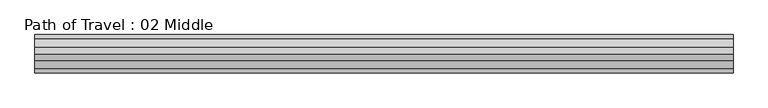
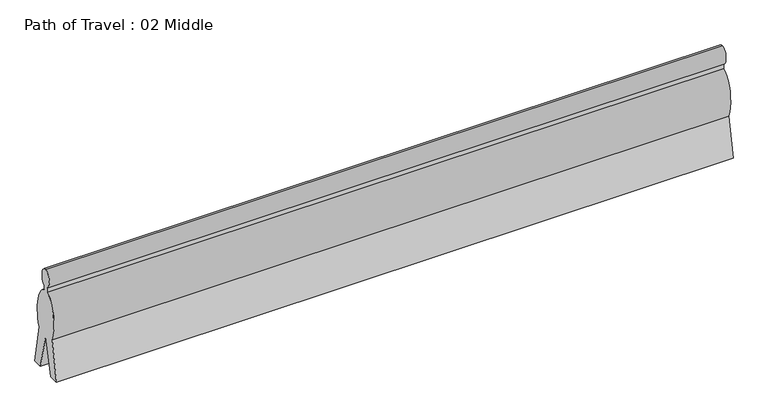
"""IFC4 building model written with IfcOpenShell, lengths in millimetres: proxy geometry, Path of Travel : 02 Middle."""

from ifc_helpers import new_model, si_unit, point, frame, origin, place, context, project, spatial, ellipse_curve, trimmed, source, transform, mapped, element, save
from ifc_brep_helpers import plane_surface, extruded_surface, advanced_brep


def path_of_travel_02_middle_3282dce8(model_context):
    return source(origin(), model_context, "Body", "AdvancedBrep", [
        advanced_brep(
        [(227.5554837, 0.0, 1727.2), (227.5554837, 42.9018657, 1436.6534209), (227.5554837, 42.9018657, 1363.4763406), (227.5554837, 184.1186263, 643.4144547), (227.5554837, 297.5699544, 0.0), (227.5554837, 145.6574193, 0.0), (227.5554837, 0.0, 584.2), (227.5554837, -145.6574193, 0.0), (227.5554837, -297.5699544, 0.0), (227.5554837, -184.1186263, 643.4144547), (227.5554837, -42.9018657, 1363.4763406), (227.5554837, -42.9018657, 1436.6534209), (11047.9554837, 0.0, 1727.2), (11047.9554837, -42.9018657, 1436.6534209), (11047.9554837, -42.9018657, 1363.4763406), (11047.9554837, -184.1186263, 643.4144547), (11047.9554837, -297.5699544, 0.0), (11047.9554837, -145.6574193, 0.0), (11047.9554837, 0.0, 584.2), (11047.9554837, 145.6574193, 0.0), (11047.9554837, 297.5699544, 0.0), (11047.9554837, 184.1186263, 643.4144547), (11047.9554837, 42.9018657, 1363.4763406), (11047.9554837, 42.9018657, 1436.6534209)],
        [
            (0, 1, ellipse_curve(frame((227.5554837, 0.0, 1574.8), z_axis=(-1.0, 0.0, 0.0), x_axis=(0.0, 0.0, 1.0)), 152.4, 101.6)),
            (1, 2),
            (2, 3, ellipse_curve(frame((227.5554837, 0.0, 914.4), z_axis=(-1.0, 0.0, 0.0), x_axis=(0.0, 0.0, -1.0)), 457.2, 228.6)),
            (3, 4),
            (4, 5),
            (5, 6),
            (6, 7),
            (7, 8),
            (8, 9),
            (9, 10, ellipse_curve(frame((227.5554837, 0.0, 914.4), z_axis=(-1.0, 0.0, 0.0), x_axis=(0.0, 0.0, -1.0)), 457.2, 228.6)),
            (10, 11),
            (11, 0, ellipse_curve(frame((227.5554837, 0.0, 1574.8), z_axis=(-1.0, 0.0, 0.0), x_axis=(0.0, 0.0, 1.0)), 152.4, 101.6)),
            (12, 13, ellipse_curve(frame((11047.9554837, 0.0, 1574.8), z_axis=(1.0, 0.0, 0.0), x_axis=(0.0, 0.0, 1.0)), 152.4, 101.6)),
            (13, 14),
            (14, 15, ellipse_curve(frame((11047.9554837, 0.0, 914.4), z_axis=(1.0, 0.0, 0.0), x_axis=(0.0, 0.0, -1.0)), 457.2, 228.6)),
            (15, 16),
            (16, 17),
            (17, 18),
            (18, 19),
            (19, 20),
            (20, 21),
            (21, 22, ellipse_curve(frame((11047.9554837, 0.0, 914.4), z_axis=(1.0, 0.0, 0.0), x_axis=(0.0, 0.0, -1.0)), 457.2, 228.6)),
            (22, 23),
            (23, 12, ellipse_curve(frame((11047.9554837, 0.0, 1574.8), z_axis=(1.0, 0.0, 0.0), x_axis=(0.0, 0.0, 1.0)), 152.4, 101.6)),
            (0, 12),
            (23, 1),
            (22, 2),
            (21, 3),
            (20, 4),
            (19, 5),
            (18, 6),
            (17, 7),
            (16, 8),
            (15, 9),
            (14, 10),
            (13, 11),
        ],
        [
            plane_surface(frame((227.5554837, 0.0, 0.0), z_axis=(-1.0, 0.0, 0.0), x_axis=(0.0, 0.0, 1.0))),
            plane_surface(frame((11047.9554837, 0.0, 0.0), z_axis=(1.0, 0.0, 0.0), x_axis=(0.0, 0.0, 1.0))),
            extruded_surface(trimmed(ellipse_curve(frame((11047.9554837, 0.0, 1574.8), z_axis=(-1.0, 0.0, 0.0), x_axis=(0.0, 0.0, 1.0)), 152.4, 101.6), [point((11047.9554837, 0.0, 1727.2))], [point((11047.9554837, 42.9018657, 1436.6534209))], True, "CARTESIAN"), (-10820.4, 0.0, 0.0), 10820.4),
            plane_surface(frame((227.5554837, 42.9018657, 1436.6534209), z_axis=(0.0, 1.0, 0.0), x_axis=(1.0, 0.0, 0.0))),
            extruded_surface(trimmed(ellipse_curve(frame((11047.9554837, 0.0, 914.4), z_axis=(-1.0, 0.0, 0.0), x_axis=(0.0, 0.0, -1.0)), 457.2, 228.6), [point((11047.9554837, 42.9018657, 1363.4763406))], [point((11047.9554837, 184.1186263, 643.4144547))], True, "CARTESIAN"), (-10820.4, 0.0, 0.0), 10820.4),
            plane_surface(frame((227.5554837, 184.1186263, 643.4144547), z_axis=(0.0, 0.9848077530122078, 0.17364817766693205), x_axis=(1.0, 0.0, 0.0))),
            plane_surface(frame((227.5554837, 297.5699544, 0.0), z_axis=(0.0, 0.0, -1.0), x_axis=(1.0, 0.0, 0.0))),
            plane_surface(frame((227.5554837, 145.6574193, 0.0), z_axis=(0.0, -0.9702957262760199, -0.2419218955995739), x_axis=(1.0, 0.0, 0.0))),
            plane_surface(frame((227.5554837, 0.0, 584.2), z_axis=(0.0, 0.9702957262759961, -0.24192189559966923), x_axis=(1.0, 0.0, 0.0))),
            plane_surface(frame((227.5554837, -145.6574193, 0.0), z_axis=(0.0, 0.0, -1.0), x_axis=(1.0, 0.0, 0.0))),
            plane_surface(frame((227.5554837, -297.5699544, 0.0), z_axis=(0.0, -0.984807753012208, 0.17364817766693066), x_axis=(1.0, 0.0, 0.0))),
            extruded_surface(trimmed(ellipse_curve(frame((11047.9554837, 0.0, 914.4), z_axis=(-1.0, 0.0, 0.0), x_axis=(0.0, 0.0, -1.0)), 457.2, 228.6), [point((11047.9554837, -184.1186263, 643.4144547))], [point((11047.9554837, -42.9018657, 1363.4763406))], True, "CARTESIAN"), (-10820.4, 0.0, 0.0), 10820.4),
            plane_surface(frame((227.5554837, -42.9018657, 1363.4763406), z_axis=(0.0, -1.0, 0.0), x_axis=(1.0, 0.0, 0.0))),
            extruded_surface(trimmed(ellipse_curve(frame((11047.9554837, 0.0, 1574.8), z_axis=(-1.0, 0.0, 0.0), x_axis=(0.0, 0.0, 1.0)), 152.4, 101.6), [point((11047.9554837, -42.9018657, 1436.6534209))], [point((11047.9554837, 0.0, 1727.2))], True, "CARTESIAN"), (-10820.4, 0.0, 0.0), 10820.4),
        ],
        [
            (0, [[1, 2, 3, 4, 5, 6, 7, 8, 9, 10, 11, 12]]),
            (1, [[13, 14, 15, 16, 17, 18, 19, 20, 21, 22, 23, 24]]),
            (2, [[-1, 25, -24, 26]]),
            (3, [[-2, -26, -23, 27]]),
            (4, [[-3, -27, -22, 28]]),
            (5, [[-4, -28, -21, 29]]),
            (6, [[-5, -29, -20, 30]]),
            (7, [[-6, -30, -19, 31]]),
            (8, [[-7, -31, -18, 32]]),
            (9, [[-8, -32, -17, 33]]),
            (10, [[-9, -33, -16, 34]]),
            (11, [[-10, -34, -15, 35]]),
            (12, [[-11, -35, -14, 36]]),
            (13, [[-12, -36, -13, -25]]),
        ],
    ),
    ])


if __name__ == "__main__":
    model = new_model("IFC4")
    model_context = context("Model", 3, world=origin())
    ifc_project = project(units=[si_unit("LENGTHUNIT", "METRE", prefix="MILLI")], contexts=[model_context])
    site = spatial("IfcSite", under=ifc_project)
    building = spatial("IfcBuilding", under=site)
    placement = place(None, origin())
    path_of_travel_02_middle_shape = path_of_travel_02_middle_3282dce8(model_context)
    element("IfcBuildingElementProxy", 1, Name="Path of Travel : 02 Middle", ObjectType="Path of Travel : 02 Middle", at=placement, inside=building, context=model_context, shape_type="MappedRepresentation", body=[
        mapped(path_of_travel_02_middle_shape, transform((0.0, 0.0, 0.0), x_axis=(1.0, 0.0, 0.0), y_axis=(0.0, 1.0, 0.0), z_axis=(0.0, 0.0, 1.0))),
    ])
    save(model, "model.ifc")

# Revit data of these elements
# Type "Path of Travel : 02 Middle"
#   Path of Egress [instance default] = 4' - 0"
#   built-in parameter 1001306 [instance default] = 4 (stored number, unit not read)
#   Dot at Start = no
#   Arrow in Middle = yes
#   Arrow at End = no
#   Egress Path = none
# Element 1 (IfcBuildingElementProxy, "Path of Travel : 02 Middle")
#   Path of Egress = 35' - 6"
#   built-in parameter 1001306 = 35.5 (stored number, unit not read)
#   Materials on its faces: "Egress Path Solid"
# Materials
#   "Egress Path Solid": class "Unassigned", colour RGB 255 128 64, transparency 0.75, Comments = "Rendering appearance not upgraded "
